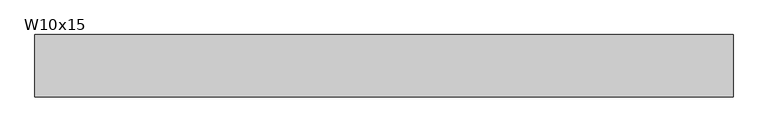
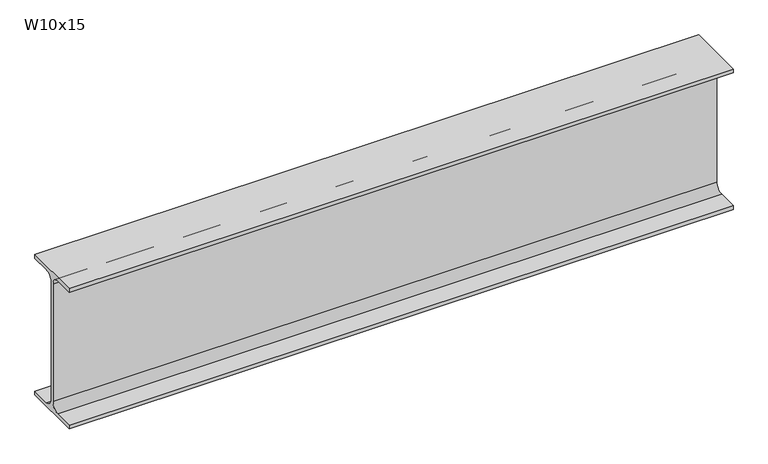
"""IFC4 building model written with IfcOpenShell, lengths in millimetres: beam geometry, RME W-Wide Flange : W10x15."""

from ifc_helpers import new_model, si_unit, point, frame, frame_2d, origin, place, context, project, spatial, polyline, circle_curve, trimmed, segment, composite_curve, outline, extrude, source, transform, mapped, element, save


def w10x15_d3763ec3(model_context):
    return source(origin(), model_context, "Body", "SweptSolid", [
        extrude(outline(composite_curve([segment(polyline([(50.8, -120.142), (50.8, -127.0), (-50.8, -127.0), (-50.8, -120.142), (-16.7005, -120.142)]), True, "CONTINUOUS"), segment(trimmed(circle_curve(frame_2d((-16.7005, -106.3625)), 13.7795), [point((-16.7005, -120.142))], [point((-2.921, -106.3625))], True, "CARTESIAN"), True, "CONTINUOUS"), segment(polyline([(-2.921, -106.3625), (-2.921, 106.3625)]), True, "CONTINUOUS"), segment(trimmed(circle_curve(frame_2d((-16.7005, 106.3625)), 13.7795), [point((-2.921, 106.3625))], [point((-16.7005, 120.142))], True, "CARTESIAN"), True, "CONTINUOUS"), segment(polyline([(-16.7005, 120.142), (-50.8, 120.142), (-50.8, 127.0), (50.8, 127.0), (50.8, 120.142), (16.7005, 120.142)]), True, "CONTINUOUS"), segment(trimmed(circle_curve(frame_2d((16.7005, 106.3625)), 13.7795), [point((16.7005, 120.142))], [point((2.921, 106.3625))], True, "CARTESIAN"), True, "CONTINUOUS"), segment(polyline([(2.921, 106.3625), (2.921, -106.3625)]), True, "CONTINUOUS"), segment(trimmed(circle_curve(frame_2d((16.7005, -106.3625)), 13.7795), [point((2.921, -106.3625))], [point((16.7005, -120.142))], True, "CARTESIAN"), True, "CONTINUOUS"), segment(polyline([(16.7005, -120.142), (50.8, -120.142)]), True, "CONTINUOUS")], self_intersect=False)), frame((-522.5686703, 0.0, 0.0), z_axis=(1.0, 0.0, 0.0), x_axis=(0.0, 1.0, 0.0)), (0.0, 0.0, 1.0), 1134.0373406),
    ])


if __name__ == "__main__":
    model = new_model("IFC4")
    model_context = context("Model", 3, world=origin())
    ifc_project = project(units=[si_unit("LENGTHUNIT", "METRE", prefix="MILLI")], contexts=[model_context])
    site = spatial("IfcSite", under=ifc_project)
    building = spatial("IfcBuilding", under=site)
    placement = place(None, origin())
    w10x15_shape = w10x15_d3763ec3(model_context)
    element("IfcBeam", 1, ObjectType="RME W-Wide Flange : W10x15", at=placement, inside=building, context=model_context, shape_type="MappedRepresentation", body=[
        mapped(w10x15_shape, transform((0.0, 0.0, 0.0), x_axis=(1.0, 0.0, 0.0), y_axis=(0.0, 1.0, 0.0), z_axis=(0.0, 0.0, 1.0))),
    ])
    save(model, "model.ifc")

# Revit data of these elements
# Type "RME W-Wide Flange : W10x15"
#   WELD P [instance default] = ""
#   WELD LE [instance default] = ""
#   WELD D [instance default] = ""
#   TOP SECTION SIZE [instance default] = ""
#   TOP SECTION LENGTH [instance default] = ""
#   REMARKS [instance default] = ""
#   REINF TYPE [instance default] = ""
#   Nominal Size = "W24"
#   End Bearing Capacity [instance default] = ""
#   BOT SECTION SIZE [instance default] = ""
#   BOT SECTION LENGTH [instance default] = ""
#   Assembly Code = "B10"
#   W = 15
#   Start Extension Calculation [instance default] = 10' - 0"
#   Start Extension [instance default] = -0' - 0 1/2"
#   End Extension Calculation [instance default] = 10' - 0"
#   End Extension [instance default] = -0' - 0 1/2"
#   Length [instance default] = 5' - 0"
#   bf = 0' - 4"
#   d = 0' - 10"
#   k = 0' - 0 13/16"
#   k2 = 0' - 0.5425"
#   tf = 0' - 0.27"
#   tw = 0' - 0.23"
#   A = 0.030625 SF
#   Structural Material [instance default] = Metal - Steel - ASTM A992
# Element 1 (IfcBeam, "RME W-Wide Flange : W10x15")
#   Length = 4' - 0.14714"
#   Materials on its faces: "Metal - Steel - ASTM A992"
# Materials
#   "Metal - Steel - ASTM A992": class "Metal", colour RGB 255 128 0, transparency 0
